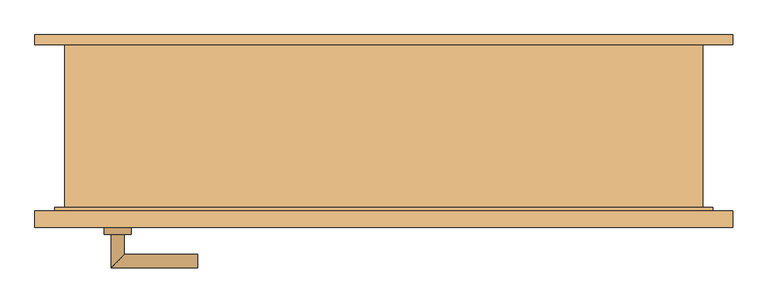
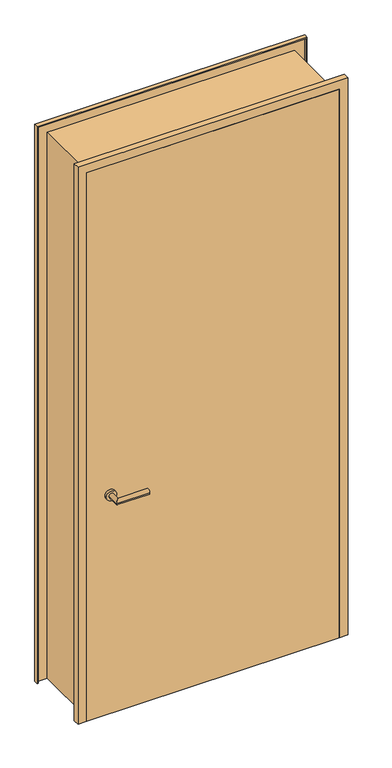
"""IFC4 building model written with IfcOpenShell, lengths in millimetres: door geometry, Drehflügel 1-flg - Variabel : Drehflügel 1-flg - Variabel."""

from ifc_helpers import new_model, si_unit, point, frame, frame_2d, origin, origin_with_axes, place, context, project, spatial, polyline, circle_curve, ellipse_curve, trimmed, segment, composite_curve, outline, extrude, faceted_brep, source, transform, mapped, element, save
from ifc_brep_helpers import plane_surface, cylinder_surface, advanced_brep


def door_8099202d(model_context):
    return source(origin(), model_context, "Body", "SolidModel", [
        advanced_brep(
        [(-410.0, -114.4346141, 900.0), (-390.0, -114.4346141, 900.0), (-390.0, -64.4346141, 900.0), (-410.0, -44.4346141, 900.0), (-280.0, -44.4346141, 900.0), (-280.0, -64.4346141, 900.0)],
        [
            (0, 1, circle_curve(frame((-400.0, -114.4346141, 900.0), z_axis=(0.0, -1.0, 0.0), x_axis=(1.0, 0.0, 0.0)), 10.0)),
            (1, 0, circle_curve(frame((-400.0, -114.4346141, 900.0), z_axis=(0.0, -1.0, 0.0), x_axis=(1.0, 0.0, 0.0)), 10.0)),
            (1, 2),
            (2, 3, ellipse_curve(frame((-400.0, -54.4346141, 900.0), z_axis=(-0.7071067811865385, -0.7071067811865565, 0.0), x_axis=(0.7071067811865563, -0.7071067811865386, 0.0)), 14.1421356, 10.0)),
            (3, 0),
            (3, 2, ellipse_curve(frame((-400.0, -54.4346141, 900.0), z_axis=(-0.7071067811865385, -0.7071067811865565, 0.0), x_axis=(0.7071067811865563, -0.7071067811865386, 0.0)), 14.1421356, 10.0)),
            (4, 5, circle_curve(frame((-280.0, -54.4346141, 900.0), z_axis=(1.0, 0.0, 0.0), x_axis=(0.0, -1.0, 0.0)), 10.0)),
            (5, 4, circle_curve(frame((-280.0, -54.4346141, 900.0), z_axis=(1.0, 0.0, 0.0), x_axis=(0.0, -1.0, 0.0)), 10.0)),
            (2, 5),
            (4, 3),
        ],
        [
            plane_surface(frame((-400.0, -114.4346141, -387.7526403), z_axis=(0.0, -1.0, 0.0), x_axis=(0.0, 0.0, 1.0))),
            cylinder_surface(frame((-400.0, -114.4346141, 900.0), z_axis=(0.0, -1.0, 0.0), x_axis=(1.0, 0.0, 0.0)), 10.0),
            plane_surface(frame((-280.0, -54.4346141, -387.7526403), z_axis=(1.0, 0.0, 0.0), x_axis=(0.0, 0.0, 1.0))),
            cylinder_surface(frame((-400.0, -54.4346141, 900.0), z_axis=(-1.0, 0.0, 0.0), x_axis=(0.0, -1.0, 0.0)), 10.0),
        ],
        [
            (0, [[1, 2]]),
            (1, [[3, 4, 5, -2]]),
            (1, [[-5, 6, -3, -1]]),
            (2, [[7, 8]]),
            (3, [[9, -7, 10, -4]]),
            (3, [[-10, -8, -9, -6]]),
        ],
    ),
        advanced_brep(
        [(-390.0, -174.4346141, 900.0), (-410.0, -174.4346141, 900.0), (-410.0, -224.4346141, 900.0), (-390.0, -204.4346141, 900.0), (-280.0, -204.4346141, 900.0), (-280.0, -224.4346141, 900.0)],
        [
            (0, 1, circle_curve(frame((-400.0, -174.4346141, 900.0), z_axis=(0.0, 1.0, 0.0), x_axis=(-1.0, 0.0, 0.0)), 10.0)),
            (1, 0, circle_curve(frame((-400.0, -174.4346141, 900.0), z_axis=(0.0, 1.0, 0.0), x_axis=(-1.0, 0.0, 0.0)), 10.0)),
            (1, 2),
            (2, 3, ellipse_curve(frame((-400.0, -214.4346141, 900.0), z_axis=(-0.7071067811865475, 0.7071067811865475, 0.0), x_axis=(0.7071067811865474, 0.7071067811865476, 0.0)), 14.1421356, 10.0)),
            (3, 0),
            (3, 2, ellipse_curve(frame((-400.0, -214.4346141, 900.0), z_axis=(-0.7071067811865475, 0.7071067811865475, 0.0), x_axis=(0.7071067811865474, 0.7071067811865476, 0.0)), 14.1421356, 10.0)),
            (4, 5, circle_curve(frame((-280.0, -214.4346141, 900.0), z_axis=(1.0, 0.0, 0.0), x_axis=(0.0, -1.0, 0.0)), 10.0)),
            (5, 4, circle_curve(frame((-280.0, -214.4346141, 900.0), z_axis=(1.0, 0.0, 0.0), x_axis=(0.0, -1.0, 0.0)), 10.0)),
            (2, 5),
            (4, 3),
        ],
        [
            plane_surface(frame((-400.0, -174.4346141, -387.7526403), z_axis=(0.0, 1.0, 0.0), x_axis=(0.0, 0.0, 1.0))),
            cylinder_surface(frame((-400.0, -174.4346141, 900.0), z_axis=(0.0, 1.0, 0.0), x_axis=(-1.0, 0.0, 0.0)), 10.0),
            plane_surface(frame((-280.0, -214.4346141, -387.7526403), z_axis=(1.0, 0.0, 0.0), x_axis=(0.0, 0.0, 1.0))),
            cylinder_surface(frame((-400.0, -214.4346141, 900.0), z_axis=(-1.0, 0.0, 0.0), x_axis=(0.0, -1.0, 0.0)), 10.0),
        ],
        [
            (0, [[1, 2]]),
            (1, [[3, 4, 5, -2]]),
            (1, [[-5, 6, -3, -1]]),
            (2, [[7, 8]]),
            (3, [[9, -7, 10, -4]]),
            (3, [[-10, -8, -9, -6]]),
        ],
    ),
        extrude(outline(composite_curve([segment(trimmed(circle_curve(frame_2d((900.0, -400.0)), 20.0), [point((900.0, -420.0))], [point((900.0, -380.0))], False, "CARTESIAN"), True, "CONTINUOUS"), segment(trimmed(circle_curve(frame_2d((900.0, -400.0)), 20.0), [point((900.0, -380.0))], [point((900.0, -420.0))], False, "CARTESIAN"), True, "CONTINUOUS")], self_intersect=False)), frame((0.0, -114.4346141, 0.0), z_axis=(0.0, 1.0, 0.0), x_axis=(0.0, 0.0, 1.0)), (0.0, 0.0, 1.0), 10.0),
        extrude(outline(composite_curve([segment(trimmed(circle_curve(frame_2d((900.0, -400.0)), 20.0), [point((900.0, -420.0))], [point((900.0, -380.0))], False, "CARTESIAN"), True, "CONTINUOUS"), segment(trimmed(circle_curve(frame_2d((900.0, -400.0)), 20.0), [point((900.0, -380.0))], [point((900.0, -420.0))], False, "CARTESIAN"), True, "CONTINUOUS")], self_intersect=False)), frame((0.0, -174.4346141, 0.0), z_axis=(0.0, 1.0, 0.0), x_axis=(0.0, 0.0, 1.0)), (0.0, 0.0, 1.0), 10.0),
        extrude(outline(polyline([(490.0, -139.4346141), (490.0, -164.4346141), (-490.0, -164.4346141), (-490.0, -139.4346141), (490.0, -139.4346141)])), origin_with_axes(), (0.0, 0.0, 1.0), 2250.0),
        faceted_brep([(524.4603207, 125.5653859, 0.0), (524.4603207, 110.5653859, 0.0), (519.4603207, 110.5653859, 0.0), (519.4603207, 120.5653859, 0.0), (480.0, 120.5653859, 0.0), (480.0, -134.4346141, 0.0), (495.0, -134.4346141, 0.0), (495.0, -159.4346141, 0.0), (519.4603207, -159.4346141, 0.0), (519.4603207, -139.4346141, 0.0), (524.4603207, -139.4346141, 0.0), (524.4603207, -164.4346141, 0.0), (490.0, -164.4346141, 0.0), (490.0, -139.4346141, 0.0), (475.0, -139.4346141, 0.0), (475.0, 125.5653859, 0.0), (475.0, 125.5653859, 2235.0), (-475.0, 125.5653859, 2235.0), (-475.0, 125.5653859, 0.0), (-524.4603207, 125.5653859, 0.0), (-524.4603207, 125.5653859, 2284.4603207), (524.4603207, 125.5653859, 2284.4603207), (475.0, -139.4346141, 2235.0), (490.0, -139.4346141, 2250.0), (-490.0, -139.4346141, 2250.0), (-490.0, -139.4346141, 0.0), (-475.0, -139.4346141, 0.0), (-475.0, -139.4346141, 2235.0), (490.0, -164.4346141, 2250.0), (524.4603207, -164.4346141, 2284.4603207), (-524.4603207, -164.4346141, 2284.4603207), (-524.4603207, -164.4346141, 0.0), (-490.0, -164.4346141, 0.0), (-490.0, -164.4346141, 2250.0), (524.4603207, -139.4346141, 2284.4603207), (519.4603207, -139.4346141, 2279.4603207), (-519.4603207, -139.4346141, 2279.4603207), (-519.4603207, -139.4346141, 0.0), (-524.4603207, -139.4346141, 0.0), (-524.4603207, -139.4346141, 2284.4603207), (519.4603207, -159.4346141, 2279.4603207), (495.0, -159.4346141, 2255.0), (-495.0, -159.4346141, 2255.0), (-495.0, -159.4346141, 0.0), (-519.4603207, -159.4346141, 0.0), (-519.4603207, -159.4346141, 2279.4603207), (495.0, -134.4346141, 2255.0), (480.0, -134.4346141, 2240.0), (-480.0, -134.4346141, 2240.0), (-480.0, -134.4346141, 0.0), (-495.0, -134.4346141, 0.0), (-495.0, -134.4346141, 2255.0), (480.0, 120.5653859, 2240.0), (519.4603207, 120.5653859, 2279.4603207), (-519.4603207, 120.5653859, 2279.4603207), (-519.4603207, 120.5653859, 0.0), (-480.0, 120.5653859, 0.0), (-480.0, 120.5653859, 2240.0), (519.4603207, 110.5653859, 2279.4603207), (524.4603207, 110.5653859, 2284.4603207), (-524.4603207, 110.5653859, 2284.4603207), (-524.4603207, 110.5653859, 0.0), (-519.4603207, 110.5653859, 0.0), (-519.4603207, 110.5653859, 2279.4603207)], [[[0, 1, 2, 3, 4, 5, 6, 7, 8, 9, 10, 11, 12, 13, 14, 15]], [[15, 16, 17, 18, 19, 20, 21, 0]], [[14, 22, 16, 15]], [[13, 23, 24, 25, 26, 27, 22, 14]], [[12, 28, 23, 13]], [[11, 29, 30, 31, 32, 33, 28, 12]], [[10, 34, 29, 11]], [[9, 35, 36, 37, 38, 39, 34, 10]], [[8, 40, 35, 9]], [[7, 41, 42, 43, 44, 45, 40, 8]], [[6, 46, 41, 7]], [[5, 47, 48, 49, 50, 51, 46, 6]], [[4, 52, 47, 5]], [[3, 53, 54, 55, 56, 57, 52, 4]], [[2, 58, 53, 3]], [[1, 59, 60, 61, 62, 63, 58, 2]], [[0, 21, 59, 1]], [[20, 19, 61, 60]], [[19, 18, 26, 25, 32, 31, 38, 37, 44, 43, 50, 49, 56, 55, 62, 61]], [[27, 26, 18, 17]], [[33, 32, 25, 24]], [[39, 38, 31, 30]], [[45, 44, 37, 36]], [[51, 50, 43, 42]], [[57, 56, 49, 48]], [[63, 62, 55, 54]], [[22, 27, 17, 16]], [[28, 33, 24, 23]], [[34, 39, 30, 29]], [[40, 45, 36, 35]], [[46, 51, 42, 41]], [[52, 57, 48, 47]], [[58, 63, 54, 53]], [[21, 20, 60, 59]]]),
    ])


if __name__ == "__main__":
    model = new_model("IFC4")
    model_context = context("Model", 3, world=origin())
    ifc_project = project(units=[si_unit("LENGTHUNIT", "METRE", prefix="MILLI")], contexts=[model_context])
    site = spatial("IfcSite", under=ifc_project)
    building = spatial("IfcBuilding", under=site)
    placement = place(None, origin())
    door_shape = door_8099202d(model_context)
    element("IfcDoor", 1, ObjectType="Drehflügel 1-flg - Variabel : Drehflügel 1-flg - Variabel", at=placement, inside=building, context=model_context, shape_type="MappedRepresentation", body=[
        mapped(door_shape, transform((0.0, 0.0, 0.0), x_axis=(1.0, 0.0, 0.0), y_axis=(0.0, 1.0, 0.0), z_axis=(0.0, 0.0, 1.0))),
    ])
    save(model, "model.ifc")

# Revit data of these elements
# Type "Drehflügel 1-flg - Variabel : Drehflügel 1-flg - Variabel"
#   Construction Type Id = "MDOOR"
#   Type Mark = "15"
#   Operation = "SingleSwingRight"
#   Keynote = "16.03"
#   Analytic Construction = "Metall"
#   Thermal Resistance (R) = 0.270117 (m²·K)/W
#   Heat Transfer Coefficient (U) = 3.7021 W/(m²·K)
#   Rough Width [instance default] = 1.000 m
#   Rough Height [instance default] = 2.360 m
#   Höhe Türgriff [instance default] = 0.900 m
#   Height [instance default] = 2.260 m
#   Fußbodenaufbau [instance default] = 0.100 m
#   Width [instance default] = 1.000 m
#   Sichtbarkeit Sturzlinien [instance default] = yes
#   Türgriff auswählen [instance default] = element 217699
#   Türgriff [instance default] = none
#   Türflügel [instance default] = none
#   Rahmen/Pfosten [instance default] = Metall - Lackiert - Grau
#   Visual Light Transmittance = 0
#   Solar Heat Gain Coefficient = 0
#   Function = (empty or 0)
#   Wall Closure = (empty or 0)
# Element 1 (IfcDoor, "Drehflügel 1-flg - Variabel : Drehflügel 1-flg - Variabel")
#   Rough Height = 2.260 m
#   Fußbodenaufbau = 0.000 m
#   Materials on its faces: "Metall - Lackiert - Grau", "Metall - Chrom", "Holz - Birke"
# Materials
#   "Metall - Lackiert - Grau": class "Farbe 1", colour RGB 98 98 98, transparency 0, Cost = 0
#   "Metall - Chrom": class "Metall", colour RGB 247 247 247, transparency 0, Cost = 0
#   "Holz - Birke": class "Holz", colour RGB 213 164 103, transparency 0, Cost = 0
